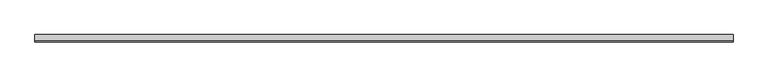
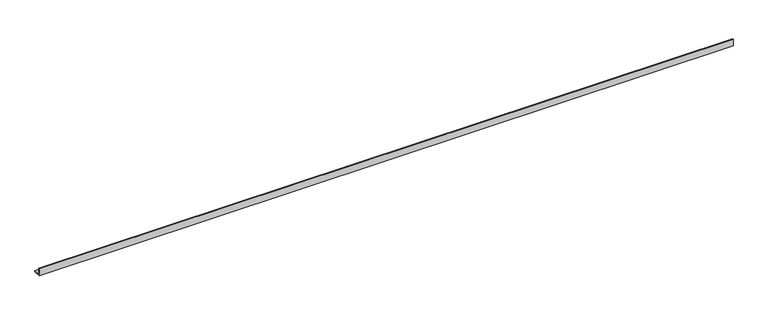
"""IFC4 building model written with IfcOpenShell, lengths in millimetres: proxy geometry, Generic Models 7:Generic Models 1:337419:Generic Models 1:337419 : Generic Models 7:Generic Models 1:337419:15 : Generic Models 7:Generic Models 1:337419:Generic Models 1:337419 : Generic Models 7:Generic Models 1:337419:301336."""

from ifc_helpers import new_model, si_unit, frame, origin, place, context, project, spatial, polyline, outline, extrude, source, transform, mapped, element, save


def generic_models_84b5536f(model_context):
    return source(origin(), model_context, "Body", "SweptSolid", [
        extrude(outline(polyline([(-536531.8913358, 8522.3945313), (-536531.8913358, 8573.1945313), (-536527.1288358, 8573.1945313), (-536527.1288358, 8527.1570313), (-536481.0913358, 8527.1570313), (-536481.0913358, 8522.3945313), (-536531.8913358, 8522.3945313)])), frame((591306.0367242, 0.0, 0.0), z_axis=(1.0, 0.0, 0.0), x_axis=(0.0, 1.0, 0.0)), (0.0, 0.0, 1.0), 4876.8),
    ])


if __name__ == "__main__":
    model = new_model("IFC4")
    model_context = context("Model", 3, world=origin())
    ifc_project = project(units=[si_unit("LENGTHUNIT", "METRE", prefix="MILLI")], contexts=[model_context])
    site = spatial("IfcSite", under=ifc_project)
    building = spatial("IfcBuilding", under=site)
    placement = place(None, origin())
    generic_models_shape = generic_models_84b5536f(model_context)
    element("IfcBuildingElementProxy", 1, Name="Generic Models 7:Generic Models 1:337419:Generic Models 1:337419 : Generic Models 7:Generic Models 1:337419:15 : Generic Models 7:Generic Models 1:337419:Generic Models 1:337419 : Generic Models 7:Generic Models 1:337419:301336", ObjectType="Generic Models 7:Generic Models 1:337419:Generic Models 1:337419 : Generic Models 7:Generic Models 1:337419:15 : Generic Models 7:Generic Models 1:337419:Generic Models 1:337419 : Generic Models 7:Generic Models 1:337419:301336", at=placement, inside=building, context=model_context, shape_type="MappedRepresentation", body=[
        mapped(generic_models_shape, transform((0.0, 0.0, 0.0), x_axis=(1.0, 0.0, 0.0), y_axis=(0.0, 1.0, 0.0), z_axis=(0.0, 0.0, 1.0))),
    ])
    save(model, "model.ifc")

# Revit data of these elements
# Type "Generic Models 7:Generic Models 1:337419:Generic Models 1:337419 : Generic Models 7:Generic Models 1:337419:15 : Generic Models 7:Generic Models 1:337419:Generic Models 1:337419 : Generic Models 7:Generic Models 1:337419:301336"
#   NameOverride = "Generic Models 7:Generic Models 1:337419:Generic Models 1:337419 : Generic Models 7:Generic Models 1:337419:301336"
#   ObjectTypeOverride = "Generic Models 1:337419 : Generic Models 7:Generic Models 1:337419"
#   Reference = "Generic Models 1"
#   Tag = "301336"
# Element 1 (IfcBuildingElementProxy, "Generic Models 7:Generic Models 1:337419:Generic Models 1:337419 : Generic Models 7:Generic Models 1:337419:15 : Generic Models 7:Generic Models 1:337419:Generic Models 1:337419 : Generic Models 7:Generic Models 1:337419:301336")
#   Materials on its faces: "GALVANIZED STEEL ANGLE (L2x2x1/4) WITH #12 GRADE 5 SCREWS @ 24\" O.C."
# Materials
#   "GALVANIZED STEEL ANGLE (L2x2x1/4) WITH #12 GRADE 5 SCREWS @ 24\" O.C.": class "Unassigned", colour RGB 210 209 208, transparency 0, Keynote = "M05121300.02", Cost = 0
